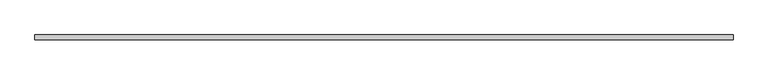
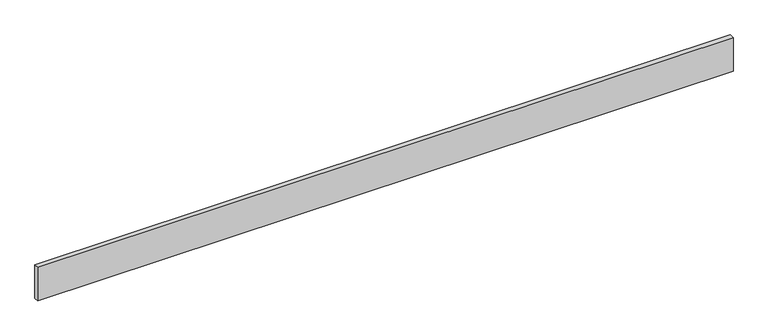
"""IFC4 building model written with IfcOpenShell, lengths in millimetres: proxy geometry, Footer 446 : Footer 446."""

from ifc_helpers import new_model, si_unit, frame, origin, place, context, project, spatial, polyline, outline, extrude, source, transform, mapped, element, save


def generic_models_91414a6d(model_context):
    return source(origin(), model_context, "Body", "SweptSolid", [
        extrude(outline(polyline([(3694.2883192, 10249.9578959), (3694.2883192, 10263.7368438), (5694.2883192, 10263.7368438), (5694.2883192, 10249.9578959), (3694.2883192, 10249.9578959)])), frame((0.0, 0.0, 40157.1476562), z_axis=(0.0, 0.0, 1.0), x_axis=(1.0, 0.0, 0.0)), (0.0, 0.0, 1.0), 101.6),
    ])


if __name__ == "__main__":
    model = new_model("IFC4")
    model_context = context("Model", 3, world=origin())
    ifc_project = project(units=[si_unit("LENGTHUNIT", "METRE", prefix="MILLI")], contexts=[model_context])
    site = spatial("IfcSite", under=ifc_project)
    building = spatial("IfcBuilding", under=site)
    placement = place(None, origin())
    generic_models_shape = generic_models_91414a6d(model_context)
    element("IfcBuildingElementProxy", 1, Name="Footer 446 : Footer 446", ObjectType="Footer 446 : Footer 446", at=placement, inside=building, context=model_context, shape_type="MappedRepresentation", body=[
        mapped(generic_models_shape, transform((0.0, 0.0, 0.0), x_axis=(1.0, 0.0, 0.0), y_axis=(0.0, 1.0, 0.0), z_axis=(0.0, 0.0, 1.0))),
    ])
    save(model, "model.ifc")

# Revit data of these elements
# Type "Footer 446 : Footer 446"
#   NameOverride = "Footer"
# Element 1 (IfcBuildingElementProxy, "Footer 446 : Footer 446")
#   Materials on its faces: "FOOTER MATERIAL TBD"
# Materials
#   "FOOTER MATERIAL TBD": class "Unassigned", colour RGB 148 103 60, transparency 0
